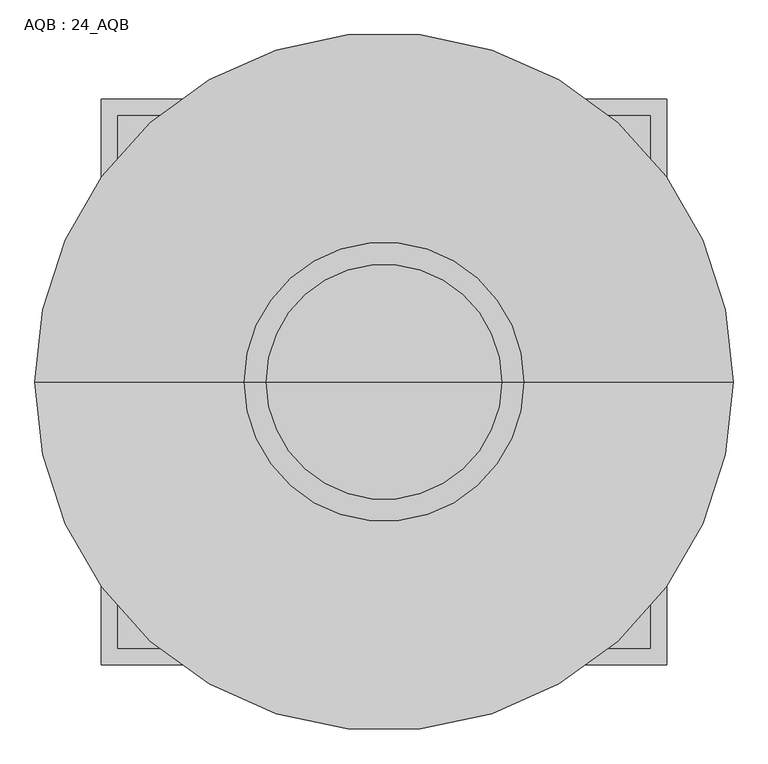
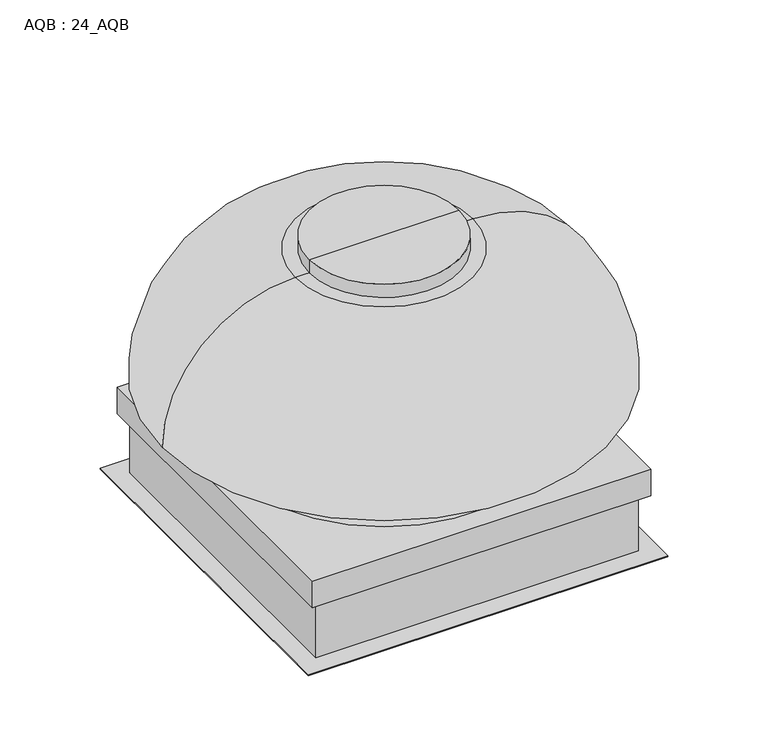
"""IFC4 building model written with IfcOpenShell, lengths in millimetres: proxy geometry, AQB : 24_AQB."""

import ifcopenshell
import ifcopenshell.guid

model = None  # the IFC model being written
_history = None  # IfcOwnerHistory: only IFC2X3 demands one
_inside = {}  # id of a spatial element -> (the spatial element, [elements in it])
_under = {}  # id of a project, library or spatial element -> (it, [spatial elements below it])
_declared = {}  # id of a project -> (the project, [libraries it declares])
_typed = {}  # id of a type object -> (the type object, [elements of that type])
_made_of = {}  # id of a material, layer set ... -> (it, [elements and type objects made of it])


def new_model(schema):
    """Start an empty IFC model of exactly this schema.

    Asked for "IFC4X3", IfcOpenShell would pick the latest addendum, in which some entities
    have other attributes; the version numbers below select the first issue.
    IFC2X3 requires an IfcOwnerHistory on every rooted entity: one is made here for all.
    """
    global model, _history
    if schema == "IFC4X3":
        model = ifcopenshell.file(schema_version=(4, 3, 0, 0))
    else:
        model = ifcopenshell.file(schema=schema)
    _inside.clear()
    _under.clear()
    _declared.clear()
    _typed.clear()
    _made_of.clear()
    _history = None
    if model.schema == "IFC2X3":
        org = make("IfcOrganization", Name="unknown")
        user = make(
            "IfcPersonAndOrganization",
            ThePerson=make("IfcPerson", FamilyName="unknown"),
            TheOrganization=org,
        )
        app = make(
            "IfcApplication",
            ApplicationDeveloper=org,
            Version="unknown",
            ApplicationFullName="unknown",
            ApplicationIdentifier="unknown",
        )
        _history = make(
            "IfcOwnerHistory",
            OwningUser=user,
            OwningApplication=app,
            ChangeAction="ADDED",
            CreationDate=0,
        )
    return model


def make(cls, **values):
    """One entity of the class cls with the attributes given. An attribute that is None is left unset."""
    return model.create_entity(
        cls, **{name: value for name, value in values.items() if value is not None}
    )


def rooted(cls, **values):
    """An entity with a GlobalId (a new one), such as an element, a storey or a relation."""
    return make(cls, GlobalId=ifcopenshell.guid.new(), OwnerHistory=_history, **values)


def si_unit(unit_type, name, prefix=None):
    """IfcSIUnit, for example si_unit("LENGTHUNIT", "METRE", prefix="MILLI")."""
    return make("IfcSIUnit", UnitType=unit_type, Prefix=prefix, Name=name)


def assignment(units):
    """IfcUnitAssignment: the units of a project."""
    return None if units is None else make("IfcUnitAssignment", Units=units)


def point(xyz):
    """IfcCartesianPoint."""
    return None if xyz is None else make("IfcCartesianPoint", Coordinates=xyz)


def direction(xyz):
    """IfcDirection."""
    return None if xyz is None else make("IfcDirection", DirectionRatios=xyz)


def frame(location, z_axis=None, x_axis=None):
    """IfcAxis2Placement3D, a coordinate frame: its origin and axes. An axis left out is left unset."""
    return make(
        "IfcAxis2Placement3D",
        Location=point(location),
        Axis=direction(z_axis),
        RefDirection=direction(x_axis),
    )


def origin():
    """The frame at (0, 0, 0) with its axes left unset."""
    return frame((0.0, 0.0, 0.0))


def place(relative_to, where):
    """IfcLocalPlacement: puts the frame where relative to a parent placement (None: the world)."""
    return make(
        "IfcLocalPlacement", PlacementRelTo=relative_to, RelativePlacement=where
    )


def context(
    kind, dimensions, precision=None, world=None, true_north=None, identifier=None
):
    """IfcGeometricRepresentationContext, for example the 3D "Model" context."""
    return make(
        "IfcGeometricRepresentationContext",
        ContextIdentifier=identifier,
        ContextType=kind,
        CoordinateSpaceDimension=dimensions,
        Precision=precision,
        WorldCoordinateSystem=world,
        TrueNorth=true_north,
    )


def project(units=None, contexts=None):
    """IfcProject with its units and contexts."""
    return rooted(
        "IfcProject",
        Name="project",
        RepresentationContexts=contexts,
        UnitsInContext=assignment(units),
    )


def spatial(cls, under=None, at=None, **own):
    """A site, building, storey or space (cls), placed at a placement, below another one or the project."""
    s = rooted(cls, ObjectPlacement=at, **own)
    if under is not None:
        _under.setdefault(under.id(), (under, []))[1].append(s)
    return s


def polyline(points):
    """IfcPolyline through the points."""
    return make("IfcPolyline", Points=[point(p) for p in points])


def circle_curve(where, radius):
    """IfcCircle in the frame where."""
    return make("IfcCircle", Position=where, Radius=radius)


def ellipse_curve(where, semi_axis1, semi_axis2):
    """IfcEllipse in the frame where."""
    return make(
        "IfcEllipse", Position=where, SemiAxis1=semi_axis1, SemiAxis2=semi_axis2
    )


def trimmed(basis, trim1, trim2, sense, master):
    """IfcTrimmedCurve: the piece of a basis curve between two trims."""
    return make(
        "IfcTrimmedCurve",
        BasisCurve=basis,
        Trim1=trim1,
        Trim2=trim2,
        SenseAgreement=sense,
        MasterRepresentation=master,
    )


def outline(outer, holes=None, kind="AREA"):
    """IfcArbitraryClosedProfileDef: a profile drawn as a closed curve; with holes, ...WithVoids."""
    if holes is None:
        return make("IfcArbitraryClosedProfileDef", ProfileType=kind, OuterCurve=outer)
    return make(
        "IfcArbitraryProfileDefWithVoids",
        ProfileType=kind,
        OuterCurve=outer,
        InnerCurves=holes,
    )


def extrude(swept, where, along, depth):
    """IfcExtrudedAreaSolid: the profile swept, set in the frame where, extruded along a direction by depth."""
    return make(
        "IfcExtrudedAreaSolid",
        SweptArea=swept,
        Position=where,
        ExtrudedDirection=direction(along),
        Depth=depth,
    )


def faces_of(points, faces, orient=None, outer=None):
    """IfcFace entities. A face is a list of loops; a loop is a list of indices into points, from 0.

    orient and outer hold one flag for each loop. By default every Orientation is true, the
    first loop of a face is its IfcFaceOuterBound and the others are IfcFaceBound.
    """
    made = []
    for i, loops in enumerate(faces):
        bounds = []
        for j, loop in enumerate(loops):
            is_outer = j == 0 if outer is None else outer[i][j]
            bounds.append(
                make(
                    "IfcFaceOuterBound" if is_outer else "IfcFaceBound",
                    Bound=make("IfcPolyLoop", Polygon=[points[k] for k in loop]),
                    Orientation=True if orient is None else orient[i][j],
                )
            )
        made.append(make("IfcFace", Bounds=bounds))
    return made


def faceted_brep(points, faces, orient=None, outer=None, voids=None):
    """IfcFacetedBrep: a solid bounded by flat faces; with voids (closed shells), ...WithVoids."""
    shared = [point(p) for p in points]
    hull = make("IfcClosedShell", CfsFaces=faces_of(shared, faces, orient, outer))
    if voids is None:
        return make("IfcFacetedBrep", Outer=hull)
    return make(
        "IfcFacetedBrepWithVoids",
        Outer=hull,
        Voids=[
            make(cls, CfsFaces=faces_of(shared, fs, o, b)) for cls, fs, o, b in voids
        ],
    )


def shape(context_of_items, identifier, shape_type, items):
    """IfcShapeRepresentation: the items that make up one representation, for example the "Body"."""
    return make(
        "IfcShapeRepresentation",
        ContextOfItems=context_of_items,
        RepresentationIdentifier=identifier,
        RepresentationType=shape_type,
        Items=items,
    )


def source(mapping_origin, context_of_items, identifier, shape_type, items):
    """IfcRepresentationMap: a shape defined once, which mapped items show again and again."""
    return make(
        "IfcRepresentationMap",
        MappingOrigin=mapping_origin,
        MappedRepresentation=shape(context_of_items, identifier, shape_type, items),
    )


def transform(
    local_origin,
    x_axis=None,
    y_axis=None,
    z_axis=None,
    scale=None,
    scale2=None,
    scale3=None,
    uniform=True,
):
    """IfcCartesianTransformationOperator3D, or its non-uniform kind. x_axis, y_axis, z_axis: its Axis1, 2, 3."""
    if uniform:
        return make(
            "IfcCartesianTransformationOperator3D",
            Axis1=direction(x_axis),
            Axis2=direction(y_axis),
            LocalOrigin=point(local_origin),
            Scale=scale,
            Axis3=direction(z_axis),
        )
    return make(
        "IfcCartesianTransformationOperator3DnonUniform",
        Axis1=direction(x_axis),
        Axis2=direction(y_axis),
        LocalOrigin=point(local_origin),
        Scale=scale,
        Axis3=direction(z_axis),
        Scale2=scale2,
        Scale3=scale3,
    )


def mapped(mapping_source, mapping_target):
    """IfcMappedItem: shows the shape of a source again, moved by a transform."""
    return make(
        "IfcMappedItem", MappingSource=mapping_source, MappingTarget=mapping_target
    )


def made_of(thing, what):
    """Note that an element or type object is made of a material, layer set ...; save() writes the relation."""
    if what is not None:
        _made_of.setdefault(what.id(), (what, []))[1].append(thing)
    return thing


def element(
    cls,
    number,
    at=None,
    inside=None,
    cuts=None,
    type_object=None,
    material=None,
    context=None,
    identifier="Body",
    shape_type=None,
    held_by="IfcProductDefinitionShape",
    body=None,
    shapes=None,
    **own,
):
    """One element of the class cls, such as IfcWall. Its Tag is "e" and its number.

    at: its placement. inside: the storey or other place that contains it. cuts: it is an
    opening in that element (IfcRelVoidsElement). A single representation is given by context,
    identifier, shape_type and body (its items); several are given by shapes. held_by: the class
    of the entity that holds the representations. save() writes the other relations.
    """
    e = rooted(cls, Tag="e%d" % number, ObjectPlacement=at, **own)
    if body is not None:
        shapes = [shape(context, identifier, shape_type, body)]
    if shapes is not None:
        e.Representation = make(held_by, Representations=shapes)
    if inside is not None:
        _inside.setdefault(inside.id(), (inside, []))[1].append(e)
    if cuts is not None:
        rooted(
            "IfcRelVoidsElement", RelatingBuildingElement=cuts, RelatedOpeningElement=e
        )
    if type_object is not None:
        _typed.setdefault(type_object.id(), (type_object, []))[1].append(e)
    return made_of(e, material)


def aggregate(whole, parts):
    """IfcRelAggregates: a whole, such as a stair, and the parts it consists of."""
    return rooted("IfcRelAggregates", RelatingObject=whole, RelatedObjects=parts)


def save(model, path):
    """Write the relations noted so far, then the file.

    IfcRelAggregates (storeys below a building ...), IfcRelContainedInSpatialStructure (elements
    in a storey), IfcRelDefinesByType, IfcRelAssociatesMaterial and IfcRelDeclares: one each for
    every whole, place, type object, material and project.
    """
    for whole, parts in _under.values():
        aggregate(whole, parts)
    for where, things in _inside.values():
        rooted(
            "IfcRelContainedInSpatialStructure",
            RelatedElements=things,
            RelatingStructure=where,
        )
    for kind, things in _typed.values():
        rooted("IfcRelDefinesByType", RelatedObjects=things, RelatingType=kind)
    for what, things in _made_of.values():
        rooted("IfcRelAssociatesMaterial", RelatedObjects=things, RelatingMaterial=what)
    for by, libraries in _declared.values():
        rooted("IfcRelDeclares", RelatingContext=by, RelatedDefinitions=libraries)
    model.write(path)


def plane_surface(at):
    """IfcPlane: the flat surface through the origin of the frame at, square to its z axis."""
    return make("IfcPlane", Position=at)


def cylinder_surface(at, radius):
    """IfcCylindricalSurface: all points at the distance radius from the z axis of the frame at."""
    return make("IfcCylindricalSurface", Position=at, Radius=radius)


def revolved_surface(curve, axis_point, axis_direction):
    """IfcSurfaceOfRevolution: the curve turned about the line through axis_point along axis_direction."""
    return make(
        "IfcSurfaceOfRevolution",
        SweptCurve=make("IfcArbitraryOpenProfileDef", ProfileType="CURVE", Curve=curve),
        AxisPosition=make("IfcAxis1Placement", Location=point(axis_point), Axis=direction(axis_direction)),
    )


def advanced_brep(points, edges, surfaces, faces):
    """IfcAdvancedBrep: a solid bounded by faces that lie on surfaces and meet in shared edges.

    An edge is (start, end): straight between two places in points (the first is 0);
    or (start, end, curve); or (start, end, curve, False) where it runs against its curve.
    A face is (place in surfaces, loops), or (place, loops, False) where it looks against
    its surface's normal. A loop lists edges by number (the first is 1), with a minus sign
    where the edge is run from its end to its start. The first loop is the outer one.
    """
    corners = [point(p) for p in points]
    vertices = [make("IfcVertexPoint", VertexGeometry=c) for c in corners]
    made = []
    for start, end, *more in edges:
        made.append(
            make(
                "IfcEdgeCurve",
                EdgeStart=vertices[start],
                EdgeEnd=vertices[end],
                EdgeGeometry=more[0] if more else make("IfcPolyline", Points=[corners[start], corners[end]]),
                SameSense=more[1] if len(more) > 1 else True,
            )
        )
    hull = []
    for where, loops, *sense in faces:
        bounds = []
        for j, loop in enumerate(loops):
            ring = [make("IfcOrientedEdge", EdgeElement=made[abs(k) - 1], Orientation=k > 0) for k in loop]
            bounds.append(
                make(
                    "IfcFaceOuterBound" if j == 0 else "IfcFaceBound",
                    Bound=make("IfcEdgeLoop", EdgeList=ring),
                    Orientation=True,
                )
            )
        hull.append(make("IfcAdvancedFace", Bounds=bounds, FaceSurface=surfaces[where], SameSense=sense[0] if sense else True))
    return make("IfcAdvancedBrep", Outer=make("IfcClosedShell", CfsFaces=hull))


def aqb_24_aqb_14a4d41b(model_context):
    return source(origin(), model_context, "Body", "SolidModel", [
        extrude(outline(polyline([(499.247472, -488.95), (-478.652528, -488.95), (-478.652528, 488.95), (499.247472, 488.95), (499.247472, -488.95)]), holes=[polyline([(-427.852528, 438.15), (-427.852528, -438.15), (448.447472, -438.15), (448.447472, 438.15), (-427.852528, 438.15)])]), frame((0.0, 0.0, -168.275), z_axis=(0.0, 0.0, 1.0), x_axis=(1.0, 0.0, 0.0)), (0.0, 0.0, 1.0), 3.175),
        extrude(outline(polyline([(-427.852528, 438.15), (448.447472, 438.15), (448.447472, -438.15), (-427.852528, -438.15), (-427.852528, 438.15)]), holes=[polyline([(410.347472, -400.05), (410.347472, 400.05), (-389.752528, 400.05), (-389.752528, -400.05), (410.347472, -400.05)])]), frame((0.0, 0.0, -168.275), z_axis=(0.0, 0.0, 1.0), x_axis=(1.0, 0.0, 0.0)), (0.0, 0.0, 1.0), 241.3),
        advanced_brep(
        [(10.297472, 0.0, 593.725), (-192.902528, 0.0, 593.725), (213.497472, 0.0, 593.725), (213.497472, 0.0, 631.825), (-192.902528, 0.0, 631.825), (10.297472, 0.0, 631.825)],
        [
            (0, 1),
            (1, 2, circle_curve(frame((10.297472, 0.0, 593.725), z_axis=(0.0, 0.0, -1.0), x_axis=(-1.0, 0.0, 0.0)), 203.2)),
            (2, 0),
            (2, 1, circle_curve(frame((10.297472, 0.0, 593.725), z_axis=(0.0, 0.0, -1.0), x_axis=(-1.0, 0.0, 0.0)), 203.2)),
            (3, 4, circle_curve(frame((10.297472, 0.0, 631.825), z_axis=(0.0, 0.0, 1.0), x_axis=(-1.0, 0.0, 0.0)), 203.2)),
            (4, 5),
            (5, 3),
            (4, 3, circle_curve(frame((10.297472, 0.0, 631.825), z_axis=(0.0, 0.0, 1.0), x_axis=(-1.0, 0.0, 0.0)), 203.2)),
            (1, 4),
            (3, 2),
        ],
        [
            plane_surface(frame((10.297472, 0.0, 593.725), z_axis=(0.0, 0.0, -1.0), x_axis=(-1.0, 0.0, 0.0))),
            plane_surface(frame((10.297472, 0.0, 631.825), z_axis=(0.0, 0.0, 1.0), x_axis=(-1.0, 0.0, 0.0))),
            cylinder_surface(frame((10.297472, 0.0, 593.725), z_axis=(0.0, 0.0, -1.0), x_axis=(-1.0, 0.0, 0.0)), 203.2),
        ],
        [
            (0, [[1, 2, 3]]),
            (0, [[-3, 4, -1]]),
            (1, [[5, 6, 7]]),
            (1, [[8, -7, -6]]),
            (2, [[-2, 9, -5, 10]]),
            (2, [[-4, -10, -8, -9]]),
        ],
    ),
        advanced_brep(
        [(10.297472, 0.0, 231.775), (-592.952528, 0.0, 231.775), (613.547472, 0.0, 231.775), (251.597472, 0.0, 593.725), (-231.002528, 0.0, 593.725), (10.297472, 0.0, 593.725)],
        [
            (0, 1),
            (1, 2, circle_curve(frame((10.297472, 0.0, 231.775), z_axis=(0.0, 0.0, -1.0), x_axis=(-1.0, 0.0, 0.0)), 603.25)),
            (2, 0),
            (2, 1, circle_curve(frame((10.297472, 0.0, 231.775), z_axis=(0.0, 0.0, -1.0), x_axis=(-1.0, 0.0, 0.0)), 603.25)),
            (3, 4, circle_curve(frame((10.297472, 0.0, 593.725), z_axis=(0.0, 0.0, 1.0), x_axis=(-1.0, 0.0, 0.0)), 241.3)),
            (4, 5),
            (5, 3),
            (4, 3, circle_curve(frame((10.297472, 0.0, 593.725), z_axis=(0.0, 0.0, 1.0), x_axis=(-1.0, 0.0, 0.0)), 241.3)),
            (1, 4, circle_curve(frame((-231.002528, 0.0, 231.775), z_axis=(0.0, 1.0, 0.0), x_axis=(1.0, 0.0, 0.0)), 361.95)),
            (3, 2, circle_curve(frame((251.597472, 0.0, 231.775), z_axis=(0.0, 1.0, 0.0), x_axis=(-1.0, 0.0, 0.0)), 361.95)),
        ],
        [
            plane_surface(frame((10.297472, 0.0, 231.775), z_axis=(0.0, 0.0, -1.0), x_axis=(-1.0, 0.0, 0.0))),
            plane_surface(frame((10.297472, 0.0, 593.725), z_axis=(0.0, 0.0, 1.0), x_axis=(-1.0, 0.0, 0.0))),
            revolved_surface(trimmed(ellipse_curve(frame((-231.002528, 0.0, 231.775), z_axis=(0.0, -1.0, 0.0), x_axis=(1.0, 0.0, 0.0)), 361.95, 361.95), [point((-231.002528, 0.0, 593.725))], [point((-592.952528, 0.0, 231.775))], True, "CARTESIAN"), (10.297472, 0.0, 593.725), (0.0, 0.0, -1.0)),
        ],
        [
            (0, [[1, 2, 3]]),
            (0, [[-3, 4, -1]]),
            (1, [[5, 6, 7]]),
            (1, [[8, -7, -6]]),
            (2, [[-2, 9, -5, 10]]),
            (2, [[-4, -10, -8, -9]]),
        ],
    ),
        advanced_brep(
        [(416.697472, 0.0, 231.775), (-396.102528, 0.0, 231.775), (10.297472, 0.0, 231.775), (416.697472, 0.0, 76.2), (-396.102528, 0.0, 76.2), (10.297472, 0.0, 76.2)],
        [
            (0, 1, circle_curve(frame((10.297472, 0.0, 231.775), z_axis=(0.0, 0.0, 1.0), x_axis=(-1.0, 0.0, 0.0)), 406.4)),
            (1, 2),
            (2, 0),
            (1, 0, circle_curve(frame((10.297472, 0.0, 231.775), z_axis=(0.0, 0.0, 1.0), x_axis=(-1.0, 0.0, 0.0)), 406.4)),
            (3, 4, circle_curve(frame((10.297472, 0.0, 76.2), z_axis=(0.0, 0.0, 1.0), x_axis=(-1.0, 0.0, 0.0)), 406.4)),
            (4, 1, circle_curve(frame((-396.102528, 0.0, 153.9875), z_axis=(0.0, -1.0, 0.0), x_axis=(1.0, 0.0, 0.0)), 77.7875)),
            (0, 3, circle_curve(frame((416.697472, 0.0, 153.9875), z_axis=(0.0, -1.0, 0.0), x_axis=(-1.0, 0.0, 0.0)), 77.7875)),
            (4, 3, circle_curve(frame((10.297472, 0.0, 76.2), z_axis=(0.0, 0.0, 1.0), x_axis=(-1.0, 0.0, 0.0)), 406.4)),
            (5, 4),
            (3, 5),
        ],
        [
            plane_surface(frame((10.297472, 0.0, 231.775), z_axis=(0.0, 0.0, 1.0), x_axis=(-1.0, 0.0, 0.0))),
            revolved_surface(trimmed(ellipse_curve(frame((-396.102528, 0.0, 153.9875), z_axis=(0.0, 1.0, 0.0), x_axis=(1.0, 0.0, 0.0)), 77.7875, 77.7875), [point((-396.102528, 0.0, 231.775))], [point((-396.102528, 0.0, 76.2))], True, "CARTESIAN"), (10.297472, 0.0, 76.2), (0.0, 0.0, -1.0)),
            plane_surface(frame((10.297472, 0.0, 76.2), z_axis=(0.0, 0.0, -1.0), x_axis=(-1.0, 0.0, 0.0))),
        ],
        [
            (0, [[1, 2, 3]]),
            (0, [[4, -3, -2]]),
            (1, [[5, 6, -1, 7]]),
            (1, [[8, -7, -4, -6]]),
            (2, [[9, -5, 10]]),
            (2, [[-10, -8, -9]]),
        ],
    ),
        faceted_brep([(470.672472, 460.375, 76.2), (-450.077528, 460.375, 76.2), (-450.077528, -460.375, 76.2), (470.672472, -460.375, 76.2), (470.672472, 460.375, 0.0), (470.672472, -460.375, 0.0), (-450.077528, -460.375, 0.0), (-450.077528, 460.375, 0.0), (467.497472, 457.2, 0.0), (-446.902528, 457.2, 0.0), (-446.902528, -457.2, 0.0), (467.497472, -457.2, 0.0), (467.497472, 457.2, 73.025), (467.497472, -457.2, 73.025), (-446.902528, -457.2, 73.025), (-446.902528, 457.2, 73.025)], [[[0, 1, 2, 3]], [[4, 5, 6, 7], [8, 9, 10, 11]], [[1, 0, 4, 7]], [[2, 1, 7, 6]], [[3, 2, 6, 5]], [[0, 3, 5, 4]], [[12, 13, 14, 15]], [[12, 15, 9, 8]], [[15, 14, 10, 9]], [[14, 13, 11, 10]], [[13, 12, 8, 11]]]),
    ])


if __name__ == "__main__":
    model = new_model("IFC4")
    model_context = context("Model", 3, world=origin())
    ifc_project = project(units=[si_unit("LENGTHUNIT", "METRE", prefix="MILLI")], contexts=[model_context])
    site = spatial("IfcSite", under=ifc_project)
    building = spatial("IfcBuilding", under=site)
    placement = place(None, origin())
    aqb_24_aqb_shape = aqb_24_aqb_14a4d41b(model_context)
    element("IfcBuildingElementProxy", 1, Name="AQB : 24_AQB", ObjectType="AQB : 24_AQB", at=placement, inside=building, context=model_context, shape_type="MappedRepresentation", body=[
        mapped(aqb_24_aqb_shape, transform((0.0, 0.0, 0.0), x_axis=(1.0, 0.0, 0.0), y_axis=(0.0, 1.0, 0.0), z_axis=(0.0, 0.0, 1.0))),
    ])
    save(model, "model.ifc")

# Revit data of these elements
# Type "AQB : 24_AQB"
#   bim-seek-source_url = ""
#   Youtube clip = ""
#   Unit Weight [instance default] = ""
#   Uniclass 2015 Name = ""
#   Uniclass 2015 Code = ""
#   Uniclass 2.0 Description = "Air Vents"
#   Uniclass 2.0 Code = "PR-94-93-xx"
#   Uniclass 1.4 Description = ""
#   Uniclass 1.4 Code = ""
#   UNSPSC Code = "40101502"
#   Technical description = ""
#   Sones [instance default] = ""
#   Region South America = "None"
#   Region Oceania = "None"
#   Region North America = "US"
#   Region Middle East = "None"
#   Region Europe = "None"
#   Region Asia = "None"
#   Region Antarctica = "None"
#   Region Africa = "None"
#   QR code = ""
#   Product group = "Exhaust"
#   Product family = "Air Condition Equipment"
#   Product data url = ""
#   Product certification = ""
#   Product SKU = "roofexhaustfan"
#   Product Guid = ""
#   OmniClass Description = ""
#   OmniClass Code = ""
#   NBS Reference Description = "Air Vents"
#   NBS Reference Code = "94-93-xx"
#   Motor RPM [instance default] = ""
#   Motor Enclosure [instance default] = ""
#   Material secondary = ""
#   Material main = "Aluminium"
#   Manufacturer name = "Loren Cook Company"
#   Manufacturer country = "United States"
#   LwA [instance default] = ""
#   Installation instructions = ""
#   IFC Classification = "Roof"
#   Fan RPM [instance default] = ""
#   EAN code = ""
#   Design country = "United States"
#   Date of publishing = "4/1/2014"
#   COBIe Type Category = ""
#   BIMobject category = "Mechanical Ventilation"
#   Brake Hp [instance default] = ""
#   Type Comments = "Downblast Propeller Exhaust Ventilator Roof Mounted/Belt Drive"
#   Motor Hp [instance default] = "0"
#   Model = "AQB"
#   Weight Net (Kg) = 0
#   T_SQ/2+.125" = 0.460375 m
#   RO/2 = 0.40005 m
#   Nominal width = 0
#   Nominal height = 0
#   RO = 0.8001 m
#   T_SQ/2 = 0.4572 m
#   T_SQ = 0.9144 m
#   D/2-(A-B) = 0.2032 m
#   C_ = 1.2065 m
#   C_/2 = 0.60325 m
#   CURB_HEIGHT [instance default] = 0.2413 m
#   BASE-.125 = 0.073025 m
#   BASE = 0.0762 m
#   B/2 = 0.115888 m
#   B-C/2 = 0.077787 m
#   B-C = 0.155575 m
#   B = 0.231775 m
#   A/2 = 0.315912 m
#   A-B = 0.40005 m
#   A-1.5" = 0.593725 m
#   A = 0.631825 m
#   4" = 0.1016 m
#   2' = 0.6096 m
#   2" = 0.0508 m
#   1" = 0.0254 m
#   0 = 0.0000 m
#   Voltage [instance default] = 0 V
#   Static Pressure [instance default] = 0.0 Pa
#   Power [instance default] = 0 W
#   Motor FLA [instance default] = 0 A
#   CFM [instance default] = 0.0 L/s
#   1.5 = 0.0381 m
#   .125 = 0.003175 m
#   -(C/2) = -0.0381 m
#   -(A/2) = -0.315912 m
#   (T_SQ/2)-2" = 0.4064 m
#   bim-seek-BOPCEditionNumber = 1
#   Edition number = 1
#   CURB [instance default] = yes
#   Phase [instance default] = 0
#   Number of Poles [instance default] = 1
#   Default Elevation = 0
#   URL = ""
#   Manufacturer = ""
